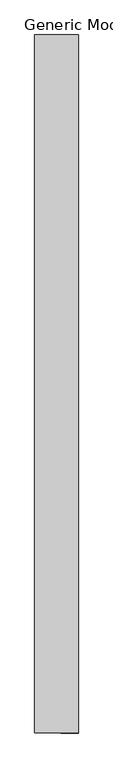
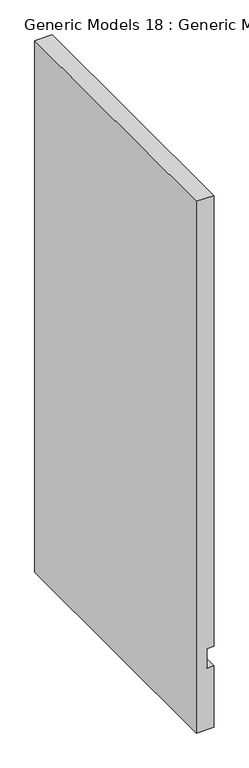
"""IFC4 building model written with IfcOpenShell, lengths in millimetres: proxy geometry, Generic Models 18 : Generic Models 1."""

from ifc_helpers import new_model, si_unit, frame, origin, place, context, project, spatial, polyline, outline, extrude, source, transform, mapped, element, save


def generic_models_18_generic_models_1_971eb1a3(model_context):
    return source(origin(), model_context, "Body", "SweptSolid", [
        extrude(outline(polyline([(7.9375, 49699.8625), (7.9375, 49776.0625), (291.1195631, 49776.0625), (291.1195631, 49745.9), (380.0195631, 49745.9), (380.0195631, 49776.0625), (2452.6875, 49776.0625), (2452.6875, 49699.8625), (7.9375, 49699.8625)])), frame((0.0, 0.0, 0.0), z_axis=(0.0, 1.0, 0.0), x_axis=(0.0, 0.0, 1.0)), (0.0, 0.0, 1.0), 1219.2),
    ])


if __name__ == "__main__":
    model = new_model("IFC4")
    model_context = context("Model", 3, world=origin())
    ifc_project = project(units=[si_unit("LENGTHUNIT", "METRE", prefix="MILLI")], contexts=[model_context])
    site = spatial("IfcSite", under=ifc_project)
    building = spatial("IfcBuilding", under=site)
    placement = place(None, origin())
    generic_models_18_generic_models_1_shape = generic_models_18_generic_models_1_971eb1a3(model_context)
    element("IfcBuildingElementProxy", 1, Name="Generic Models 18 : Generic Models 1", ObjectType="Generic Models 18 : Generic Models 1", at=placement, inside=building, context=model_context, shape_type="MappedRepresentation", body=[
        mapped(generic_models_18_generic_models_1_shape, transform((0.0, 0.0, 0.0), x_axis=(1.0, 0.0, 0.0), y_axis=(0.0, 1.0, 0.0), z_axis=(0.0, 0.0, 1.0))),
    ])
    save(model, "model.ifc")

# Revit data of these elements
# Element 1 (IfcBuildingElementProxy, "Generic Models 18 : Generic Models 1")
#   Materials on its faces: "(S) SOUND BATT. INSULATION (THICKNESS TO MATCH WALL DEPTH)"
# Materials
#   "(S) SOUND BATT. INSULATION (THICKNESS TO MATCH WALL DEPTH)": class "Unassigned", colour RGB 255 255 255, transparency 0, Cost = 0
